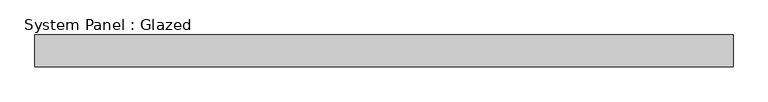
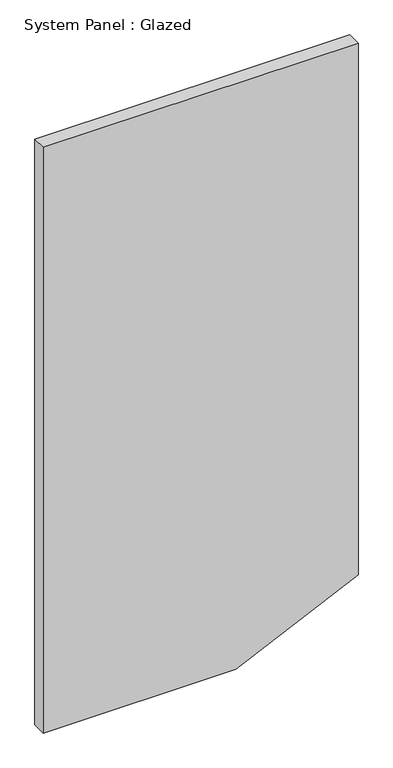
"""IFC4 building model written with IfcOpenShell, lengths in millimetres: plate geometry, System Panel : Glazed."""

from ifc_helpers import new_model, si_unit, frame, origin, place, context, project, spatial, polyline, outline, extrude, source, transform, mapped, element, save


def system_panel_glazed_d54c78e3(model_context):
    return source(origin(), model_context, "Body", "SweptSolid", [
        extrude(outline(polyline([(0.0, -550.0006382), (0.0, 122.8354585), (199.1901838, 550.0006382), (2163.3463373, 550.0006382), (2163.3463373, -550.0006382), (0.0, -550.0006382)])), frame((0.0, -25.0, 0.0), z_axis=(0.0, 1.0, 0.0), x_axis=(0.0, 0.0, 1.0)), (0.0, 0.0, 1.0), 50.0),
    ])


if __name__ == "__main__":
    model = new_model("IFC4")
    model_context = context("Model", 3, world=origin())
    ifc_project = project(units=[si_unit("LENGTHUNIT", "METRE", prefix="MILLI")], contexts=[model_context])
    site = spatial("IfcSite", under=ifc_project)
    building = spatial("IfcBuilding", under=site)
    placement = place(None, origin())
    system_panel_glazed_shape = system_panel_glazed_d54c78e3(model_context)
    element("IfcPlate", 1, ObjectType="System Panel : Glazed", at=placement, inside=building, context=model_context, shape_type="MappedRepresentation", body=[
        mapped(system_panel_glazed_shape, transform((0.0, 0.0, 0.0), x_axis=(1.0, 0.0, 0.0), y_axis=(0.0, 1.0, 0.0), z_axis=(0.0, 0.0, 1.0))),
    ])
    save(model, "model.ifc")

# Revit data of these elements
# Type "System Panel : Glazed"
#   Type Mark = "CW-GLASS"
# Element 1 (IfcPlate, "System Panel : Glazed")
#   Materials on its faces: "Glass_Clear"
# Materials
#   "Glass_Clear": class "Glass", colour RGB 128 128 255, transparency 0.8, Comments = "Rendering appearance not upgraded ", Cost = 0
